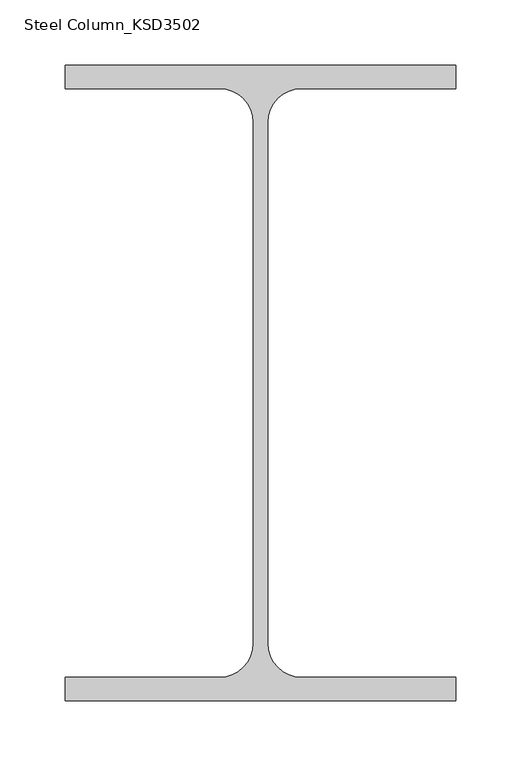
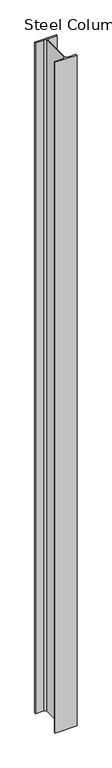
"""IFC4 building model written with IfcOpenShell, lengths in millimetres: column geometry, Steel Column_KSD3502 : H_SC_ASC_H-488×300x11x18."""

from ifc_helpers import new_model, si_unit, point, frame, frame_2d, origin, place, context, project, spatial, polyline, circle_curve, trimmed, segment, composite_curve, outline, extrude, source, transform, mapped, element, save


def steel_column_ksd3502_bd22218f(model_context):
    return source(origin(), model_context, "Body", "SweptSolid", [
        extrude(outline(composite_curve([segment(polyline([(150.0, 244.0), (150.0, 226.0), (31.5, 226.0)]), True, "CONTINUOUS"), segment(trimmed(circle_curve(frame_2d((31.5, 200.0)), 26.0), [point((31.5, 226.0))], [point((5.5, 200.0))], True, "CARTESIAN"), True, "CONTINUOUS"), segment(polyline([(5.5, 200.0), (5.5, -200.0)]), True, "CONTINUOUS"), segment(trimmed(circle_curve(frame_2d((31.5, -200.0)), 26.0), [point((5.5, -200.0))], [point((31.5, -226.0))], True, "CARTESIAN"), True, "CONTINUOUS"), segment(polyline([(31.5, -226.0), (150.0, -226.0), (150.0, -244.0), (-150.0, -244.0), (-150.0, -226.0), (-31.5, -226.0)]), True, "CONTINUOUS"), segment(trimmed(circle_curve(frame_2d((-31.5, -200.0)), 26.0), [point((-31.5, -226.0))], [point((-5.5, -200.0))], True, "CARTESIAN"), True, "CONTINUOUS"), segment(polyline([(-5.5, -200.0), (-5.5, 200.0)]), True, "CONTINUOUS"), segment(trimmed(circle_curve(frame_2d((-31.5, 200.0)), 26.0), [point((-5.5, 200.0))], [point((-31.5, 226.0))], True, "CARTESIAN"), True, "CONTINUOUS"), segment(polyline([(-31.5, 226.0), (-150.0, 226.0), (-150.0, 244.0), (150.0, 244.0)]), True, "CONTINUOUS")], self_intersect=False)), frame((0.0, 0.0, 7538.9720055), z_axis=(0.0, 0.0, 1.0), x_axis=(1.0, 0.0, 0.0)), (0.0, 0.0, 1.0), 9761.0),
    ])


if __name__ == "__main__":
    model = new_model("IFC4")
    model_context = context("Model", 3, world=origin())
    ifc_project = project(units=[si_unit("LENGTHUNIT", "METRE", prefix="MILLI")], contexts=[model_context])
    site = spatial("IfcSite", under=ifc_project)
    building = spatial("IfcBuilding", under=site)
    placement = place(None, origin())
    steel_column_ksd3502_shape = steel_column_ksd3502_bd22218f(model_context)
    element("IfcColumn", 1, ObjectType="Steel Column_KSD3502 : H_SC_ASC_H-488×300x11x18", at=placement, inside=building, context=model_context, shape_type="MappedRepresentation", body=[
        mapped(steel_column_ksd3502_shape, transform((0.0, 0.0, 0.0), x_axis=(1.0, 0.0, 0.0), y_axis=(0.0, 1.0, 0.0), z_axis=(0.0, 0.0, 1.0))),
    ])
    save(model, "model.ifc")

# Revit data of these elements
# Type "Steel Column_KSD3502 : H_SC_ASC_H-488×300x11x18"
#   Width = 30.0 cm
#   Web Thickness = 1.1 cm
#   Web Fillet = 2.6 cm
#   Warping Constant = 4473230.0 cm⁶
#   Torsional Moment of Inertia = 137.492 cm⁴
#   Section Area = 163.5 cm²
#   Plastic Modulus weak axis = 830.0 cm³
#   Plastic Modulus strong axis = 3230.0 cm³
#   Perimeter = 1.27 m²/m
#   Nominal Weight = 128.00 kgf/m
#   Moment of Inertia weak axis = 8110.00 cm⁴
#   Moment of Inertia strong axis = 71000.00 cm⁴
#   Height = 48.8 cm
#   Flange Thickness = 1.8 cm
#   Elastic Modulus weak axis = 541.0 cm³
#   Elastic Modulus strong axis = 2910.0 cm³
#   Centroid Vertical = 24.4 cm
#   Centroid Horizontal = 15.0 cm
#   Bolt Spacing = 13.97 cm
#   Structural Material [instance default] = Steel, 45-345
#   Section Name Key = ""
#   Assembly Code = ""
# Element 1 (IfcColumn, "Steel Column_KSD3502 : H_SC_ASC_H-488×300x11x18")
#   Structural Material = none
# Materials
#   "Steel, 45-345": class "Metal", colour RGB 189 187 185, transparency 0, Description = "Steel 345 MPa", Cost = 0
